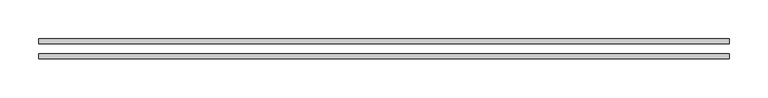
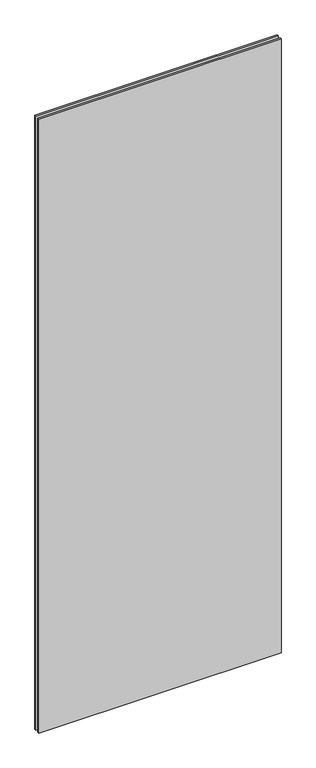
"""IFC4 building model written with IfcOpenShell, lengths in millimetres: proxy geometry, Window glass:Window glass:300352:Window glass:300352 : Window glass:Window glass:300352:300073:Window glass:300352:Window glass:300352 : Window glass:Window glass:300352:300073 : Window glass:Window glass:300352:Window glass:300352 : Window glass:Window glass:300352:300073:1 : Window glass:Window glass:300352:Window glass:300352 : Window glass:Window glass:300352:300073:Window glass:300352:Window glass:300352 : Window glass:Window glass:300352:300073 : Window glass:Window glass:300352:Window glass:300352 : Window glass:Window glass:300352:300073:300061."""

from ifc_helpers import new_model, si_unit, frame, origin, place, context, project, spatial, polyline, outline, extrude, source, transform, mapped, element, save


def generic_models_10c51317(model_context):
    return source(origin(), model_context, "Body", "SweptSolid", [
        extrude(outline(polyline([(593690.1661787, -579048.3332724), (592803.3447692, -579048.3332724), (592803.3447692, -579041.9832724), (593690.1661787, -579041.9832724), (593690.1661787, -579048.3332724)])), frame((0.0, 0.0, 70.3749752), z_axis=(0.0, 0.0, 1.0), x_axis=(1.0, 0.0, 0.0)), (0.0, 0.0, 1.0), 2377.2967003),
        extrude(outline(polyline([(593690.1661787, -579029.2832724), (592803.3447692, -579029.2832724), (592803.3447692, -579022.9332724), (593690.1661787, -579022.9332724), (593690.1661787, -579029.2832724)])), frame((0.0, 0.0, 70.3749752), z_axis=(0.0, 0.0, 1.0), x_axis=(1.0, 0.0, 0.0)), (0.0, 0.0, 1.0), 2377.2967003),
    ])


if __name__ == "__main__":
    model = new_model("IFC4")
    model_context = context("Model", 3, world=origin())
    ifc_project = project(units=[si_unit("LENGTHUNIT", "METRE", prefix="MILLI")], contexts=[model_context])
    site = spatial("IfcSite", under=ifc_project)
    building = spatial("IfcBuilding", under=site)
    placement = place(None, origin())
    generic_models_shape = generic_models_10c51317(model_context)
    element("IfcBuildingElementProxy", 1, Name="Window glass:Window glass:300352:Window glass:300352 : Window glass:Window glass:300352:300073:Window glass:300352:Window glass:300352 : Window glass:Window glass:300352:300073 : Window glass:Window glass:300352:Window glass:300352 : Window glass:Window glass:300352:300073:1 : Window glass:Window glass:300352:Window glass:300352 : Window glass:Window glass:300352:300073:Window glass:300352:Window glass:300352 : Window glass:Window glass:300352:300073 : Window glass:Window glass:300352:Window glass:300352 : Window glass:Window glass:300352:300073:300061", ObjectType="Window glass:Window glass:300352:Window glass:300352 : Window glass:Window glass:300352:300073:Window glass:300352:Window glass:300352 : Window glass:Window glass:300352:300073 : Window glass:Window glass:300352:Window glass:300352 : Window glass:Window glass:300352:300073:1 : Window glass:Window glass:300352:Window glass:300352 : Window glass:Window glass:300352:300073:Window glass:300352:Window glass:300352 : Window glass:Window glass:300352:300073 : Window glass:Window glass:300352:Window glass:300352 : Window glass:Window glass:300352:300073:300061", at=placement, inside=building, context=model_context, shape_type="MappedRepresentation", body=[
        mapped(generic_models_shape, transform((0.0, 0.0, 0.0), x_axis=(1.0, 0.0, 0.0), y_axis=(0.0, 1.0, 0.0), z_axis=(0.0, 0.0, 1.0))),
    ])
    save(model, "model.ifc")

# Revit data of these elements
# Type "Window glass:Window glass:300352:Window glass:300352 : Window glass:Window glass:300352:300073:Window glass:300352:Window glass:300352 : Window glass:Window glass:300352:300073 : Window glass:Window glass:300352:Window glass:300352 : Window glass:Window glass:300352:300073:1 : Window glass:Window glass:300352:Window glass:300352 : Window glass:Window glass:300352:300073:Window glass:300352:Window glass:300352 : Window glass:Window glass:300352:300073 : Window glass:Window glass:300352:Window glass:300352 : Window glass:Window glass:300352:300073:300061"
#   NameOverride = "Window glass:Window glass:300352:Window glass:300352 : Window glass:Window glass:300352:300073:Window glass:300352:Window glass:300352 : Window glass:Window glass:300352:300073 : Window glass:Window glass:300352:Window glass:300352 : Window glass:Window glass:300352:300073:300061"
#   ObjectTypeOverride = "Window glass:300352:Window glass:300352 : Window glass:Window glass:300352:300073 : Window glass:Window glass:300352:Window glass:300352 : Window glass:Window glass:300352:300073"
#   Reference = "Window glass"
#   Tag = "300061"
# Element 1 (IfcBuildingElementProxy, "Window glass:Window glass:300352:Window glass:300352 : Window glass:Window glass:300352:300073:Window glass:300352:Window glass:300352 : Window glass:Window glass:300352:300073 : Window glass:Window glass:300352:Window glass:300352 : Window glass:Window glass:300352:300073:1 : Window glass:Window glass:300352:Window glass:300352 : Window glass:Window glass:300352:300073:Window glass:300352:Window glass:300352 : Window glass:Window glass:300352:300073 : Window glass:Window glass:300352:Window glass:300352 : Window glass:Window glass:300352:300073:300061")
#   Materials on its faces: "INSULATED LOW-E GLAZING (SEE ELEVATIONS FOR U-FACTOR, SHGC, & LT)"
# Materials
#   "INSULATED LOW-E GLAZING (SEE ELEVATIONS FOR U-FACTOR, SHGC, & LT)": class "Unassigned", colour RGB 84 171 255, transparency 0, Cost = 0
